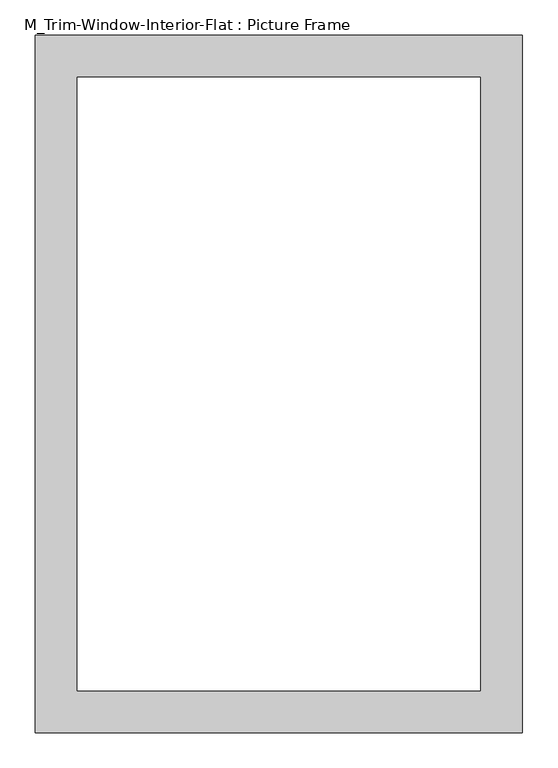
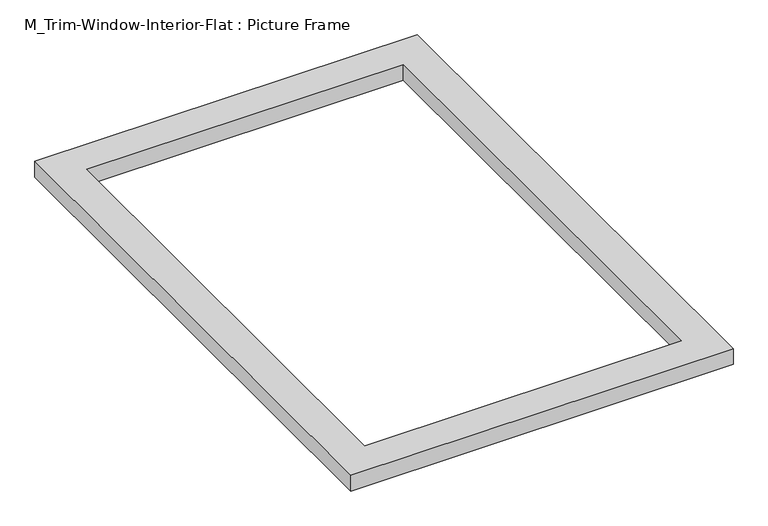
"""IFC4 building model written with IfcOpenShell, lengths in millimetres: proxy geometry, M_Trim-Window-Interior-Flat : Picture Frame."""

from ifc_helpers import new_model, si_unit, origin, origin_with_axes, place, context, project, spatial, polyline, outline, extrude, source, transform, mapped, element, save


def m_trim_window_interior_flat_picture_frame_0a41e60c(model_context):
    return source(origin(), model_context, "Body", "SweptSolid", [
        extrude(outline(polyline([(347.3, 47.3), (347.3, -947.3), (-347.3, -947.3), (-347.3, 47.3), (347.3, 47.3)]), holes=[polyline([(287.3, -12.7), (-287.3, -12.7), (-287.3, -887.3), (287.3, -887.3), (287.3, -12.7)])]), origin_with_axes(), (0.0, 0.0, 1.0), 30.0),
    ])


if __name__ == "__main__":
    model = new_model("IFC4")
    model_context = context("Model", 3, world=origin())
    ifc_project = project(units=[si_unit("LENGTHUNIT", "METRE", prefix="MILLI")], contexts=[model_context])
    site = spatial("IfcSite", under=ifc_project)
    building = spatial("IfcBuilding", under=site)
    placement = place(None, origin())
    m_trim_window_interior_flat_picture_frame_shape = m_trim_window_interior_flat_picture_frame_0a41e60c(model_context)
    element("IfcBuildingElementProxy", 1, Name="M_Trim-Window-Interior-Flat : Picture Frame", ObjectType="M_Trim-Window-Interior-Flat : Picture Frame", at=placement, inside=building, context=model_context, shape_type="MappedRepresentation", body=[
        mapped(m_trim_window_interior_flat_picture_frame_shape, transform((0.0, 0.0, 0.0), x_axis=(1.0, 0.0, 0.0), y_axis=(0.0, 1.0, 0.0), z_axis=(0.0, 0.0, 1.0))),
    ])
    save(model, "model.ifc")

# Revit data of these elements
# Type "M_Trim-Window-Interior-Flat : Picture Frame"
#   Trim Thickness_Picture Frame = 3 cm
#   Trim Width = 6 cm
#   Trim Thickness_with Sill = 2 cm
#   Sill Thickness = 3 cm
#   Opening Width [instance default] = 60 cm
#   Opening Height [instance default] = 90 cm
#   Default Elevation = 120 cm
#   Sill = no
#   Picture Frame = yes
#   Trim Material [instance default] = none
# Element 1 (IfcBuildingElementProxy, "M_Trim-Window-Interior-Flat : Picture Frame")
#   Trim Material = Wood - Stained
#   Materials on its faces: "Wood - Stained"
# Materials
#   "Wood - Stained": class "Wood", colour RGB 173 132 96, transparency 0, Cost = 0
